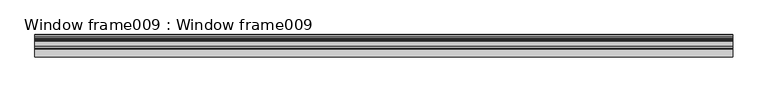
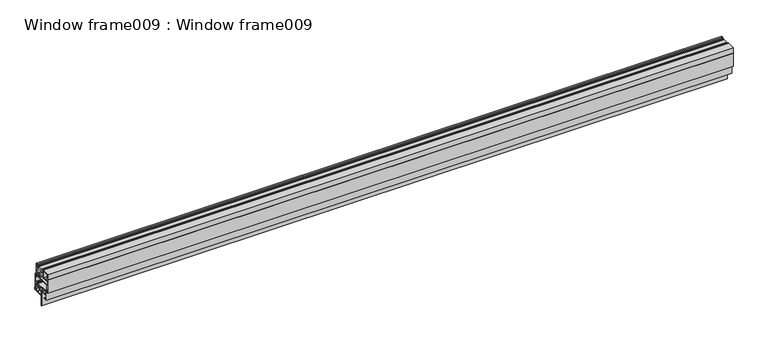
"""IFC4 building model written with IfcOpenShell, lengths in millimetres: proxy geometry, Window frame009 : Window frame009."""

from ifc_helpers import new_model, si_unit, frame, origin, place, context, project, spatial, polyline, outline, extrude, source, transform, mapped, element, save


def window_frame009_window_frame009_a827a080(model_context):
    return source(origin(), model_context, "Body", "SweptSolid", [
        extrude(outline(polyline([(-4391.3816761, 41136.035647), (-4392.5557884, 41136.035647), (-4393.2183155, 41138.6258645), (-4393.2183155, 41140.4872274), (-4392.5826763, 41143.3492036), (-4391.2293113, 41143.3492036), (-4390.80557, 41140.8903107), (-4388.579356, 41140.8903107), (-4388.579356, 41138.4773107), (-4390.8062639, 41138.4773107), (-4391.3816761, 41136.035647)])), frame((12383.0178845, 0.0, 0.0), z_axis=(1.0, 0.0, 0.0), x_axis=(0.0, 1.0, 0.0)), (0.0, 0.0, 1.0), 2000.0),
        extrude(outline(polyline([(-4421.006836, 41142.8132608), (-4419.8327236, 41142.8132608), (-4419.1701966, 41140.2230433), (-4419.1701966, 41138.3616804), (-4419.8058357, 41135.4997042), (-4421.1592007, 41135.4997042), (-4421.582942, 41137.9585971), (-4423.809156, 41137.9585971), (-4423.809156, 41140.3715971), (-4421.5822482, 41140.3715971), (-4421.006836, 41142.8132608)])), frame((12383.0178845, 0.0, 0.0), z_axis=(1.0, 0.0, 0.0), x_axis=(0.0, 1.0, 0.0)), (0.0, 0.0, 1.0), 2000.0),
        extrude(outline(polyline([(-4437.893456, 41085.2746969), (-4438.7250364, 41085.2746969), (-4438.7250364, 41088.2229435), (-4442.020956, 41088.2229435), (-4442.020956, 41089.4167435), (-4438.7250364, 41089.4167435), (-4438.7250364, 41092.7920791), (-4437.893456, 41092.7920791), (-4437.893456, 41085.2746969)])), frame((12383.0178845, 0.0, 0.0), z_axis=(1.0, 0.0, 0.0), x_axis=(0.0, 1.0, 0.0)), (0.0, 0.0, 1.0), 2000.0),
        extrude(outline(polyline([(-4386.725156, 41108.8241278), (-4385.8935756, 41108.8241278), (-4385.8935756, 41105.8758812), (-4382.597656, 41105.8758812), (-4382.597656, 41104.6820812), (-4385.8935756, 41104.6820812), (-4385.8935756, 41101.3067456), (-4386.725156, 41101.3067456), (-4386.725156, 41108.8241278)])), frame((12383.0178845, 0.0, 0.0), z_axis=(1.0, 0.0, 0.0), x_axis=(0.0, 1.0, 0.0)), (0.0, 0.0, 1.0), 2000.0),
        extrude(outline(polyline([(-4391.233656, 41059.8002812), (-4391.233656, 41061.8322812), (-4382.775456, 41061.8322812), (-4382.775456, 41072.9828812), (-4386.585456, 41072.9828812), (-4386.585456, 41077.0795922), (-4385.1624461, 41077.0795922), (-4385.1624461, 41075.0595907), (-4382.775456, 41075.0595907), (-4382.775456, 41084.5652812), (-4385.1630564, 41084.5652812), (-4385.1630564, 41082.7603386), (-4386.585456, 41082.7603386), (-4386.585456, 41084.5652812), (-4388.2121134, 41084.5652812), (-4388.2121134, 41086.5972812), (-4385.137656, 41086.5972812), (-4385.137656, 41103.4114927), (-4383.8766375, 41103.4114927), (-4383.8766375, 41102.5230812), (-4382.597656, 41102.5230812), (-4382.597656, 41107.6030812), (-4383.867656, 41107.6030812), (-4383.867656, 41106.6118864), (-4385.137656, 41106.6118864), (-4385.137656, 41108.8730812), (-4380.743456, 41108.8730812), (-4380.743456, 41059.8002812), (-4391.233656, 41059.8002812)])), frame((12383.0178845, 0.0, 0.0), z_axis=(1.0, 0.0, 0.0), x_axis=(0.0, 1.0, 0.0)), (0.0, 0.0, 1.0), 2000.0),
        extrude(outline(polyline([(-4401.266656, 41122.7668812), (-4403.438356, 41122.7668812), (-4403.438356, 41124.1384812), (-4399.8657732, 41124.1384812), (-4399.8657732, 41120.9634812), (-4398.1379436, 41120.9634812), (-4398.1379436, 41118.9314848), (-4402.727156, 41118.9314848), (-4402.727156, 41109.3810812), (-4400.1707468, 41109.3810812), (-4400.1707468, 41110.6262983), (-4398.917156, 41110.6262983), (-4398.917156, 41107.3490812), (-4439.480956, 41107.3490812), (-4439.480956, 41090.5029615), (-4440.7741228, 41090.5029615), (-4440.7741228, 41091.4098371), (-4442.020956, 41091.4098371), (-4442.020956, 41086.3460249), (-4440.7748957, 41086.3460249), (-4440.7748957, 41087.3430341), (-4439.480956, 41087.3430341), (-4439.480956, 41085.0732812), (-4443.875156, 41085.0732812), (-4443.875156, 41125.7894812), (-4440.4256318, 41125.7894812), (-4441.843156, 41122.9946349), (-4441.843156, 41120.9634812), (-4401.266656, 41120.9634812), (-4401.266656, 41122.7668812)]), holes=[polyline([(-4441.335156, 41110.5240812), (-4404.759156, 41110.5240812), (-4404.759156, 41117.7884812), (-4441.335156, 41117.7884812), (-4441.335156, 41110.5240812)])]), frame((12383.0178845, 0.0, 0.0), z_axis=(1.0, 0.0, 0.0), x_axis=(0.0, 1.0, 0.0)), (0.0, 0.0, 1.0), 2000.0),
        extrude(outline(polyline([(-4394.5782015, 41130.5392812), (-4392.8129015, 41129.0133897), (-4392.8129015, 41124.2421179), (-4391.119356, 41124.2421179), (-4391.119356, 41120.9634812), (-4397.9374172, 41120.9634812), (-4397.9374172, 41124.6608634), (-4404.8507959, 41124.6608634), (-4404.8507959, 41122.8121723), (-4418.894256, 41122.7922812), (-4418.894256, 41130.5392812), (-4394.5782015, 41130.5392812)])), frame((12383.0178845, 0.0, 0.0), z_axis=(1.0, 0.0, 0.0), x_axis=(0.0, 1.0, 0.0)), (0.0, 0.0, 1.0), 2000.0),
        extrude(outline(polyline([(12383.0178845, -4412.569656), (12383.0178845, -4399.793456), (14383.0178845, -4399.793456), (14383.0178845, -4412.569656), (12383.0178845, -4412.569656)])), frame((0.0, 0.0, 41130.5392812), z_axis=(0.0, 0.0, 1.0), x_axis=(1.0, 0.0, 0.0)), (0.0, 0.0, 1.0), 9.525),
        extrude(outline(polyline([(-4388.757156, 41107.3490812), (-4392.5458804, 41107.3490812), (-4392.5458804, 41110.6399091), (-4391.3246088, 41110.6399091), (-4391.3246088, 41109.3810812), (-4388.757156, 41109.3810812), (-4388.757156, 41118.9314848), (-4393.3545557, 41118.9314848), (-4393.3545557, 41120.9634812), (-4391.119356, 41120.9634812), (-4391.119356, 41137.7526563), (-4389.8595438, 41137.7526563), (-4389.8595438, 41136.8892812), (-4388.579356, 41136.8892812), (-4388.579356, 41141.9692812), (-4389.8771983, 41141.9692812), (-4389.8771983, 41140.9853376), (-4391.119356, 41140.9853376), (-4391.119356, 41143.2392812), (-4386.725156, 41143.2392812), (-4386.725156, 41102.5230812), (-4388.757156, 41102.5230812), (-4388.757156, 41107.3490812)])), frame((12383.0178845, 0.0, 0.0), z_axis=(1.0, 0.0, 0.0), x_axis=(0.0, 1.0, 0.0)), (0.0, 0.0, 1.0), 2000.0),
        extrude(outline(polyline([(-4394.2018007, 41075.0148812), (-4394.2018007, 41077.0795922), (-4392.935456, 41077.0795922), (-4392.935456, 41072.9828812), (-4412.4934569, 41072.9828809), (-4412.493456, 41059.7803485), (-4412.493456, 41029.4527485), (-4414.068256, 41029.4527485), (-4414.068256, 41072.9828812), (-4435.861456, 41072.9828812), (-4435.861456, 41061.8322812), (-4427.403256, 41061.8322812), (-4427.403256, 41059.8002812), (-4437.893456, 41059.8002812), (-4437.893456, 41091.4232812), (-4434.4847393, 41091.4232812), (-4435.861456, 41088.8575235), (-4435.861456, 41086.5972812), (-4395.206798, 41086.5972812), (-4395.206798, 41088.4006812), (-4398.1443306, 41088.4006812), (-4398.1443306, 41089.7722812), (-4393.9081469, 41089.7722812), (-4393.9081469, 41086.5972812), (-4392.1562439, 41086.5972812), (-4392.1562439, 41084.5652812), (-4396.745456, 41084.5652812), (-4396.745456, 41075.0148812), (-4394.2018007, 41075.0148812)]), holes=[polyline([(-4405.734973, 41083.4222812), (-4405.734973, 41084.5652812), (-4414.0647917, 41084.5652812), (-4414.0647917, 41083.4222812), (-4417.9612513, 41083.4222812), (-4417.9612513, 41084.5652812), (-4422.4459887, 41084.5652812), (-4422.4459887, 41083.4222812), (-4431.3263584, 41083.4222812), (-4431.3263584, 41084.5652812), (-4435.353456, 41084.5652812), (-4435.353456, 41075.0148812), (-4431.372099, 41075.0148812), (-4431.372099, 41076.1578812), (-4427.4516669, 41076.1578812), (-4427.4516669, 41075.0148812), (-4417.8881903, 41075.0148812), (-4417.8881903, 41076.1578812), (-4412.1857462, 41076.1578812), (-4412.1857462, 41075.0148812), (-4402.4143687, 41075.0148812), (-4402.4143687, 41076.1578812), (-4398.777456, 41076.1578812), (-4398.777456, 41083.4222812), (-4405.734973, 41083.4222812)])]), frame((12383.0178845, 0.0, 0.0), z_axis=(1.0, 0.0, 0.0), x_axis=(0.0, 1.0, 0.0)), (0.0, 0.0, 1.0), 2000.0),
        extrude(outline(polyline([(-4443.875156, 41143.2392812), (-4421.2567683, 41143.2392812), (-4421.2567683, 41141.0305189), (-4422.4955855, 41141.0305189), (-4422.4955855, 41141.9596265), (-4423.809156, 41141.9596265), (-4423.809156, 41136.8892812), (-4422.462986, 41136.8892812), (-4422.462986, 41137.786775), (-4421.2893706, 41137.786775), (-4421.2893706, 41135.6031583), (-4423.809156, 41135.6031583), (-4423.809156, 41122.7922812), (-4401.266656, 41122.7668812), (-4401.266656, 41121.3952812), (-4425.206156, 41121.3952812), (-4425.206156, 41141.8422812), (-4442.478156, 41141.8422812), (-4442.478156, 41127.1864812), (-4439.0524426, 41127.1864812), (-4439.0524426, 41122.0996946), (-4439.8585701, 41122.0996946), (-4441.3535819, 41123.5459379), (-4440.3603471, 41125.7894812), (-4443.875156, 41125.7894812), (-4443.875156, 41143.2392812)])), frame((12383.0178845, 0.0, 0.0), z_axis=(1.0, 0.0, 0.0), x_axis=(0.0, 1.0, 0.0)), (0.0, 0.0, 1.0), 2000.0),
        extrude(outline(polyline([(-4412.493456, 41028.0502812), (-4412.493456, 41059.8002812), (-4380.743456, 41059.8002812), (-4380.743456, 41066.1502812), (-4379.727456, 41066.1502812), (-4379.727456, 41058.7842812), (-4411.477456, 41058.7842812), (-4411.477456, 41028.0502812), (-4412.493456, 41028.0502812)])), frame((12383.0178845, 0.0, 0.0), z_axis=(1.0, 0.0, 0.0), x_axis=(0.0, 1.0, 0.0)), (0.0, 0.0, 1.0), 2000.0),
    ])


if __name__ == "__main__":
    model = new_model("IFC4")
    model_context = context("Model", 3, world=origin())
    ifc_project = project(units=[si_unit("LENGTHUNIT", "METRE", prefix="MILLI")], contexts=[model_context])
    site = spatial("IfcSite", under=ifc_project)
    building = spatial("IfcBuilding", under=site)
    placement = place(None, origin())
    window_frame009_window_frame009_shape = window_frame009_window_frame009_a827a080(model_context)
    element("IfcBuildingElementProxy", 1, Name="Window frame009 : Window frame009", ObjectType="Window frame009 : Window frame009", at=placement, inside=building, context=model_context, shape_type="MappedRepresentation", body=[
        mapped(window_frame009_window_frame009_shape, transform((0.0, 0.0, 0.0), x_axis=(1.0, 0.0, 0.0), y_axis=(0.0, 1.0, 0.0), z_axis=(0.0, 0.0, 1.0))),
    ])
    save(model, "model.ifc")

# Revit data of these elements
# Type "Window frame009 : Window frame009"
#   NameOverride = "Window frame009"
# Element 1 (IfcBuildingElementProxy, "Window frame009 : Window frame009")
#   Materials on its faces: "FLEETWOOD SERIES 250-T-01 CASEMENT WINDOW FRAME"
# Materials
#   "FLEETWOOD SERIES 250-T-01 CASEMENT WINDOW FRAME": class "Unassigned", colour RGB 128 128 128, transparency 0
